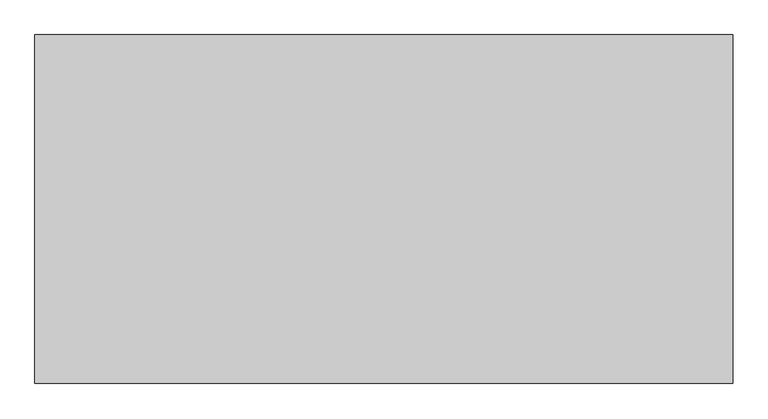
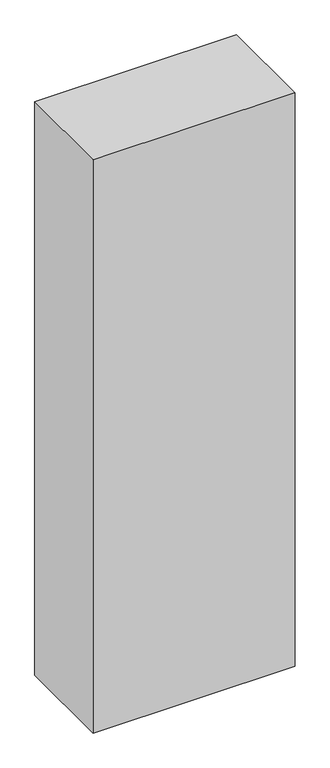
"""IFC4 building model written with IfcOpenShell, lengths in millimetres: proxy geometry, Space Planning Box_hec : Space Planning Box_hec."""

from ifc_helpers import new_model, si_unit, origin, origin_with_axes, place, context, project, spatial, polyline, outline, extrude, source, transform, mapped, element, save


def generic_models_da00a96f(model_context):
    return source(origin(), model_context, "Body", "SweptSolid", [
        extrude(outline(polyline([(1000.0, 500.0), (1000.0, -500.0), (-1000.0, -500.0), (-1000.0, 500.0), (1000.0, 500.0)])), origin_with_axes(), (0.0, 0.0, 1.0), 6000.0),
    ])


if __name__ == "__main__":
    model = new_model("IFC4")
    model_context = context("Model", 3, world=origin())
    ifc_project = project(units=[si_unit("LENGTHUNIT", "METRE", prefix="MILLI")], contexts=[model_context])
    site = spatial("IfcSite", under=ifc_project)
    building = spatial("IfcBuilding", under=site)
    placement = place(None, origin())
    generic_models_shape = generic_models_da00a96f(model_context)
    element("IfcBuildingElementProxy", 1, Name="Space Planning Box_hec : Space Planning Box_hec", ObjectType="Space Planning Box_hec : Space Planning Box_hec", at=placement, inside=building, context=model_context, shape_type="MappedRepresentation", body=[
        mapped(generic_models_shape, transform((0.0, 0.0, 0.0), x_axis=(1.0, 0.0, 0.0), y_axis=(0.0, 1.0, 0.0), z_axis=(0.0, 0.0, 1.0))),
    ])
    save(model, "model.ifc")

# Revit data of these elements
# Type "Space Planning Box_hec : Space Planning Box_hec"
#   Type Comments = "..."
#   Room Name [instance default] = "?"
#   Interior Finish [instance default] = ""
#   Exterior Finish [instance default] = ""
#   Department [instance default] = ""
#   Assembly Code = "..."
#   Width [instance default] = 1524 mm
#   Program Area [instance default] = 0.00 m²
#   Length [instance default] = 1524 mm
#   Height [instance default] = 1524 mm
#   Area [instance default] = 2.32258 m²
#   Fill Color [instance default] = Cyan
#   Default Elevation = 0
# Element 1 (IfcBuildingElementProxy, "Space Planning Box_hec : Space Planning Box_hec")
#   Room Name = "Corridor"
#   Interior Finish = "IF2-1"
#   Exterior Finish = "EF1"
#   Department = "AR"
#   Width = 2000 mm
#   Length = 1000 mm
#   Height = 6000 mm
#   Area = 2.00 m²
#   Materials on its faces: "Cyan"
# Materials
#   "Cyan": class "Generic", colour RGB 0 255 255, transparency 0.2, Cost = 0
